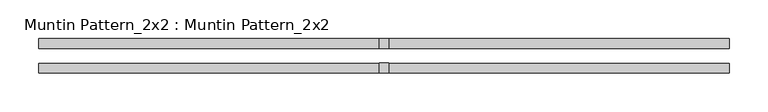
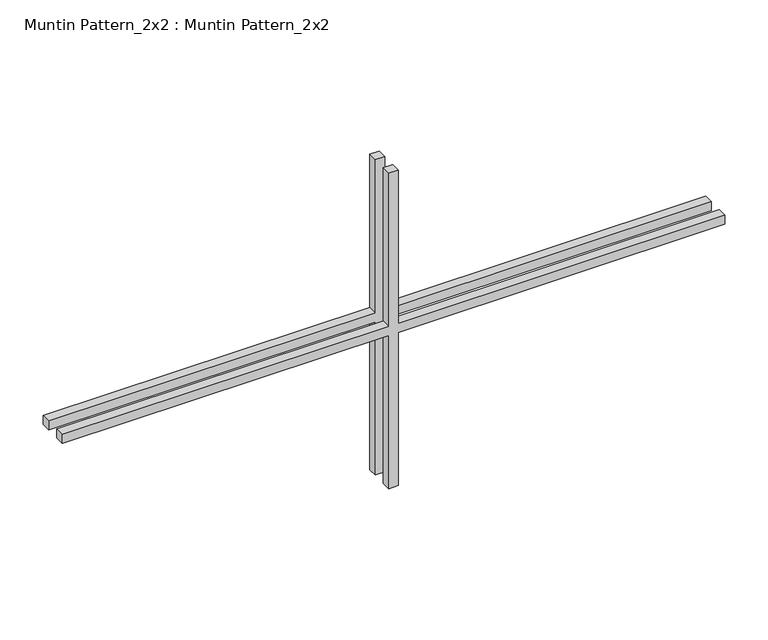
"""IFC4 building model written with IfcOpenShell, lengths in millimetres: proxy geometry, Muntin Pattern_2x2 : Muntin Pattern_2x2."""

import ifcopenshell
import ifcopenshell.guid

model = None  # the IFC model being written
_history = None  # IfcOwnerHistory: only IFC2X3 demands one
_inside = {}  # id of a spatial element -> (the spatial element, [elements in it])
_under = {}  # id of a project, library or spatial element -> (it, [spatial elements below it])
_declared = {}  # id of a project -> (the project, [libraries it declares])
_typed = {}  # id of a type object -> (the type object, [elements of that type])
_made_of = {}  # id of a material, layer set ... -> (it, [elements and type objects made of it])


def new_model(schema):
    """Start an empty IFC model of exactly this schema.

    Asked for "IFC4X3", IfcOpenShell would pick the latest addendum, in which some entities
    have other attributes; the version numbers below select the first issue.
    IFC2X3 requires an IfcOwnerHistory on every rooted entity: one is made here for all.
    """
    global model, _history
    if schema == "IFC4X3":
        model = ifcopenshell.file(schema_version=(4, 3, 0, 0))
    else:
        model = ifcopenshell.file(schema=schema)
    _inside.clear()
    _under.clear()
    _declared.clear()
    _typed.clear()
    _made_of.clear()
    _history = None
    if model.schema == "IFC2X3":
        org = make("IfcOrganization", Name="unknown")
        user = make(
            "IfcPersonAndOrganization",
            ThePerson=make("IfcPerson", FamilyName="unknown"),
            TheOrganization=org,
        )
        app = make(
            "IfcApplication",
            ApplicationDeveloper=org,
            Version="unknown",
            ApplicationFullName="unknown",
            ApplicationIdentifier="unknown",
        )
        _history = make(
            "IfcOwnerHistory",
            OwningUser=user,
            OwningApplication=app,
            ChangeAction="ADDED",
            CreationDate=0,
        )
    return model


def make(cls, **values):
    """One entity of the class cls with the attributes given. An attribute that is None is left unset."""
    return model.create_entity(
        cls, **{name: value for name, value in values.items() if value is not None}
    )


def rooted(cls, **values):
    """An entity with a GlobalId (a new one), such as an element, a storey or a relation."""
    return make(cls, GlobalId=ifcopenshell.guid.new(), OwnerHistory=_history, **values)


def si_unit(unit_type, name, prefix=None):
    """IfcSIUnit, for example si_unit("LENGTHUNIT", "METRE", prefix="MILLI")."""
    return make("IfcSIUnit", UnitType=unit_type, Prefix=prefix, Name=name)


def assignment(units):
    """IfcUnitAssignment: the units of a project."""
    return None if units is None else make("IfcUnitAssignment", Units=units)


def point(xyz):
    """IfcCartesianPoint."""
    return None if xyz is None else make("IfcCartesianPoint", Coordinates=xyz)


def direction(xyz):
    """IfcDirection."""
    return None if xyz is None else make("IfcDirection", DirectionRatios=xyz)


def frame(location, z_axis=None, x_axis=None):
    """IfcAxis2Placement3D, a coordinate frame: its origin and axes. An axis left out is left unset."""
    return make(
        "IfcAxis2Placement3D",
        Location=point(location),
        Axis=direction(z_axis),
        RefDirection=direction(x_axis),
    )


def origin():
    """The frame at (0, 0, 0) with its axes left unset."""
    return frame((0.0, 0.0, 0.0))


def place(relative_to, where):
    """IfcLocalPlacement: puts the frame where relative to a parent placement (None: the world)."""
    return make(
        "IfcLocalPlacement", PlacementRelTo=relative_to, RelativePlacement=where
    )


def context(
    kind, dimensions, precision=None, world=None, true_north=None, identifier=None
):
    """IfcGeometricRepresentationContext, for example the 3D "Model" context."""
    return make(
        "IfcGeometricRepresentationContext",
        ContextIdentifier=identifier,
        ContextType=kind,
        CoordinateSpaceDimension=dimensions,
        Precision=precision,
        WorldCoordinateSystem=world,
        TrueNorth=true_north,
    )


def project(units=None, contexts=None):
    """IfcProject with its units and contexts."""
    return rooted(
        "IfcProject",
        Name="project",
        RepresentationContexts=contexts,
        UnitsInContext=assignment(units),
    )


def spatial(cls, under=None, at=None, **own):
    """A site, building, storey or space (cls), placed at a placement, below another one or the project."""
    s = rooted(cls, ObjectPlacement=at, **own)
    if under is not None:
        _under.setdefault(under.id(), (under, []))[1].append(s)
    return s


def polyline(points):
    """IfcPolyline through the points."""
    return make("IfcPolyline", Points=[point(p) for p in points])


def outline(outer, holes=None, kind="AREA"):
    """IfcArbitraryClosedProfileDef: a profile drawn as a closed curve; with holes, ...WithVoids."""
    if holes is None:
        return make("IfcArbitraryClosedProfileDef", ProfileType=kind, OuterCurve=outer)
    return make(
        "IfcArbitraryProfileDefWithVoids",
        ProfileType=kind,
        OuterCurve=outer,
        InnerCurves=holes,
    )


def extrude(swept, where, along, depth):
    """IfcExtrudedAreaSolid: the profile swept, set in the frame where, extruded along a direction by depth."""
    return make(
        "IfcExtrudedAreaSolid",
        SweptArea=swept,
        Position=where,
        ExtrudedDirection=direction(along),
        Depth=depth,
    )


def shape(context_of_items, identifier, shape_type, items):
    """IfcShapeRepresentation: the items that make up one representation, for example the "Body"."""
    return make(
        "IfcShapeRepresentation",
        ContextOfItems=context_of_items,
        RepresentationIdentifier=identifier,
        RepresentationType=shape_type,
        Items=items,
    )


def source(mapping_origin, context_of_items, identifier, shape_type, items):
    """IfcRepresentationMap: a shape defined once, which mapped items show again and again."""
    return make(
        "IfcRepresentationMap",
        MappingOrigin=mapping_origin,
        MappedRepresentation=shape(context_of_items, identifier, shape_type, items),
    )


def transform(
    local_origin,
    x_axis=None,
    y_axis=None,
    z_axis=None,
    scale=None,
    scale2=None,
    scale3=None,
    uniform=True,
):
    """IfcCartesianTransformationOperator3D, or its non-uniform kind. x_axis, y_axis, z_axis: its Axis1, 2, 3."""
    if uniform:
        return make(
            "IfcCartesianTransformationOperator3D",
            Axis1=direction(x_axis),
            Axis2=direction(y_axis),
            LocalOrigin=point(local_origin),
            Scale=scale,
            Axis3=direction(z_axis),
        )
    return make(
        "IfcCartesianTransformationOperator3DnonUniform",
        Axis1=direction(x_axis),
        Axis2=direction(y_axis),
        LocalOrigin=point(local_origin),
        Scale=scale,
        Axis3=direction(z_axis),
        Scale2=scale2,
        Scale3=scale3,
    )


def mapped(mapping_source, mapping_target):
    """IfcMappedItem: shows the shape of a source again, moved by a transform."""
    return make(
        "IfcMappedItem", MappingSource=mapping_source, MappingTarget=mapping_target
    )


def made_of(thing, what):
    """Note that an element or type object is made of a material, layer set ...; save() writes the relation."""
    if what is not None:
        _made_of.setdefault(what.id(), (what, []))[1].append(thing)
    return thing


def element(
    cls,
    number,
    at=None,
    inside=None,
    cuts=None,
    type_object=None,
    material=None,
    context=None,
    identifier="Body",
    shape_type=None,
    held_by="IfcProductDefinitionShape",
    body=None,
    shapes=None,
    **own,
):
    """One element of the class cls, such as IfcWall. Its Tag is "e" and its number.

    at: its placement. inside: the storey or other place that contains it. cuts: it is an
    opening in that element (IfcRelVoidsElement). A single representation is given by context,
    identifier, shape_type and body (its items); several are given by shapes. held_by: the class
    of the entity that holds the representations. save() writes the other relations.
    """
    e = rooted(cls, Tag="e%d" % number, ObjectPlacement=at, **own)
    if body is not None:
        shapes = [shape(context, identifier, shape_type, body)]
    if shapes is not None:
        e.Representation = make(held_by, Representations=shapes)
    if inside is not None:
        _inside.setdefault(inside.id(), (inside, []))[1].append(e)
    if cuts is not None:
        rooted(
            "IfcRelVoidsElement", RelatingBuildingElement=cuts, RelatedOpeningElement=e
        )
    if type_object is not None:
        _typed.setdefault(type_object.id(), (type_object, []))[1].append(e)
    return made_of(e, material)


def aggregate(whole, parts):
    """IfcRelAggregates: a whole, such as a stair, and the parts it consists of."""
    return rooted("IfcRelAggregates", RelatingObject=whole, RelatedObjects=parts)


def save(model, path):
    """Write the relations noted so far, then the file.

    IfcRelAggregates (storeys below a building ...), IfcRelContainedInSpatialStructure (elements
    in a storey), IfcRelDefinesByType, IfcRelAssociatesMaterial and IfcRelDeclares: one each for
    every whole, place, type object, material and project.
    """
    for whole, parts in _under.values():
        aggregate(whole, parts)
    for where, things in _inside.values():
        rooted(
            "IfcRelContainedInSpatialStructure",
            RelatedElements=things,
            RelatingStructure=where,
        )
    for kind, things in _typed.values():
        rooted("IfcRelDefinesByType", RelatedObjects=things, RelatingType=kind)
    for what, things in _made_of.values():
        rooted("IfcRelAssociatesMaterial", RelatedObjects=things, RelatingMaterial=what)
    for by, libraries in _declared.values():
        rooted("IfcRelDeclares", RelatingContext=by, RelatedDefinitions=libraries)
    model.write(path)


def muntin_pattern_2x2_muntin_pattern_2x2_39bd07d8(model_context):
    return source(origin(), model_context, "Body", "SweptSolid", [
        extrude(outline(polyline([(230.1875, -6.35), (230.1875, -444.5), (217.4875, -444.5), (217.4875, -6.35), (0.0, -6.35), (0.0, 6.35), (217.4875, 6.35), (217.4875, 444.5), (230.1875, 444.5), (230.1875, 6.35), (447.675, 6.35), (447.675, -6.35), (230.1875, -6.35)])), frame((0.0, -22.225, 0.0), z_axis=(0.0, 1.0, 0.0), x_axis=(0.0, 0.0, 1.0)), (0.0, 0.0, 1.0), 12.7),
        extrude(outline(polyline([(230.1875, -6.35), (230.1875, -444.5), (217.4875, -444.5), (217.4875, -6.35), (0.0, -6.35), (0.0, 6.35), (217.4875, 6.35), (217.4875, 444.5), (230.1875, 444.5), (230.1875, 6.35), (447.675, 6.35), (447.675, -6.35), (230.1875, -6.35)])), frame((0.0, 9.525, 0.0), z_axis=(0.0, 1.0, 0.0), x_axis=(0.0, 0.0, 1.0)), (0.0, 0.0, 1.0), 12.7),
    ])


if __name__ == "__main__":
    model = new_model("IFC4")
    model_context = context("Model", 3, world=origin())
    ifc_project = project(units=[si_unit("LENGTHUNIT", "METRE", prefix="MILLI")], contexts=[model_context])
    site = spatial("IfcSite", under=ifc_project)
    building = spatial("IfcBuilding", under=site)
    placement = place(None, origin())
    muntin_pattern_2x2_muntin_pattern_2x2_shape = muntin_pattern_2x2_muntin_pattern_2x2_39bd07d8(model_context)
    element("IfcBuildingElementProxy", 1, Name="Muntin Pattern_2x2 : Muntin Pattern_2x2", ObjectType="Muntin Pattern_2x2 : Muntin Pattern_2x2", at=placement, inside=building, context=model_context, shape_type="MappedRepresentation", body=[
        mapped(muntin_pattern_2x2_muntin_pattern_2x2_shape, transform((0.0, 0.0, 0.0), x_axis=(1.0, 0.0, 0.0), y_axis=(0.0, 1.0, 0.0), z_axis=(0.0, 0.0, 1.0))),
    ])
    save(model, "model.ifc")

# Revit data of these elements
# Type "Muntin Pattern_2x2 : Muntin Pattern_2x2"
#   Width [instance default] = 4' - 0"
#   Thickness = 0' - 0 1/2"
#   Height [instance default] = 4' - 0"
#   Distance = 0' - 0 3/4"
#   Interior Material [instance default] = none
#   Exterior Material [instance default] = none
# Element 1 (IfcBuildingElementProxy, "Muntin Pattern_2x2 : Muntin Pattern_2x2")
#   Width = 2' - 11"
#   Height = 1' - 5 5/8"
#   Interior Material = Wood - Stained
#   Exterior Material = Clad - White
#   Materials on its faces: "Clad - White", "Wood - Stained"
# Materials
#   "Clad - White": class "Wood", colour RGB 242 242 238, transparency 0, Cost = 0
#   "Wood - Stained": class "Wood", colour RGB 224 178 126, transparency 0, Cost = 0
